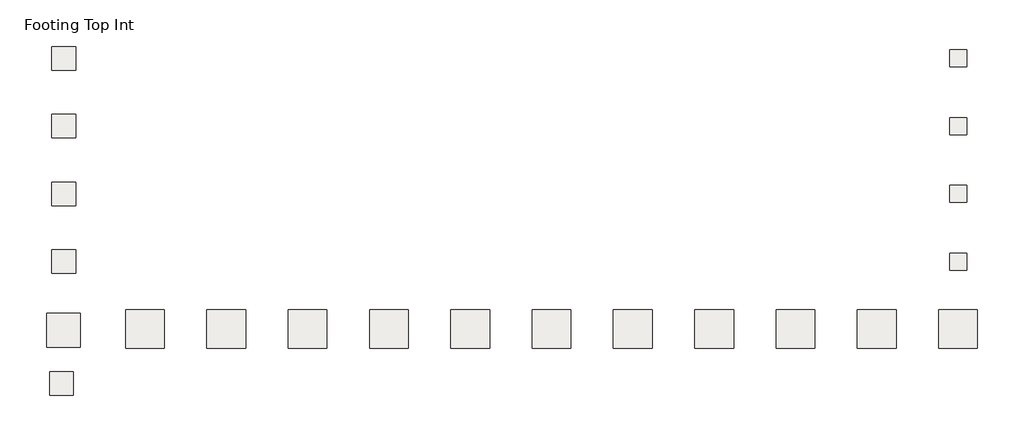
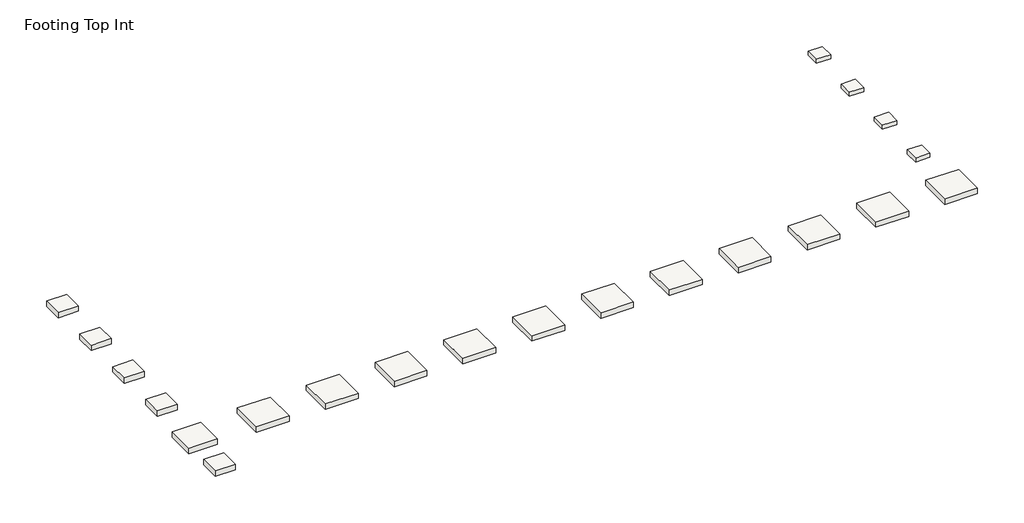
# One storey: 21 slabs.
"""IFC4 building model written with IfcOpenShell, lengths in millimetres."""

from ifc_helpers import new_model, si_unit, frame, origin, place, context, project, spatial, polyline, outline, extrude, element, save

model = new_model("IFC4")

# Units and contexts
model_context = context("Model", 3, world=origin())
ifc_project = project(units=[si_unit("LENGTHUNIT", "METRE", prefix="MILLI")], contexts=[model_context])

# Site, building, storey
site = spatial("IfcSite", under=ifc_project)
building = spatial("IfcBuilding", under=site)
storey = spatial("IfcBuildingStorey", under=building, Name="Footing Top Int", Elevation=-304.8)

# Slabs
placement = place(None, origin())
element("IfcSlab", 1, ObjectType="Footing-Rectangular : F10", at=placement, inside=storey, context=model_context, shape_type="SweptSolid", body=[
    extrude(outline(polyline([(321699.0398264, -566249.8913841), (324747.0398264, -566249.8913841), (324747.0398264, -569297.8913841), (321699.0398264, -569297.8913841), (321699.0398264, -566249.8913841)])), frame((0.0, 0.0, -914.4), z_axis=(0.0, 0.0, 1.0), x_axis=(1.0, 0.0, 0.0)), (0.0, 0.0, 1.0), 609.6),
])
element("IfcSlab", 2, ObjectType="Footing-Rectangular : F11", at=placement, inside=storey, context=model_context, shape_type="SweptSolid", body=[
    extrude(outline(polyline([(328849.1398264, -565913.3414082), (332354.3398264, -565913.3414082), (332354.3398264, -569418.5414082), (328849.1398264, -569418.5414082), (328849.1398264, -565913.3414082)])), frame((0.0, 0.0, -914.4), z_axis=(0.0, 0.0, 1.0), x_axis=(1.0, 0.0, 0.0)), (0.0, 0.0, 1.0), 609.6),
])
element("IfcSlab", 3, ObjectType="Footing-Rectangular : F11", at=placement, inside=storey, context=model_context, shape_type="SweptSolid", body=[
    extrude(outline(polyline([(336202.4398264, -565913.3414082), (339707.6398264, -565913.3414082), (339707.6398264, -569418.5414082), (336202.4398264, -569418.5414082), (336202.4398264, -565913.3414082)])), frame((0.0, 0.0, -914.4), z_axis=(0.0, 0.0, 1.0), x_axis=(1.0, 0.0, 0.0)), (0.0, 0.0, 1.0), 609.6),
])
element("IfcSlab", 4, ObjectType="Footing-Rectangular : F11", at=placement, inside=storey, context=model_context, shape_type="SweptSolid", body=[
    extrude(outline(polyline([(343555.7398264, -565913.3414082), (347060.9398264, -565913.3414082), (347060.9398264, -569418.5414082), (343555.7398264, -569418.5414082), (343555.7398264, -565913.3414082)])), frame((0.0, 0.0, -914.4), z_axis=(0.0, 0.0, 1.0), x_axis=(1.0, 0.0, 0.0)), (0.0, 0.0, 1.0), 609.6),
])
element("IfcSlab", 5, ObjectType="Footing-Rectangular : F11", at=placement, inside=storey, context=model_context, shape_type="SweptSolid", body=[
    extrude(outline(polyline([(350909.0398264, -565913.3414082), (354414.2398264, -565913.3414082), (354414.2398264, -569418.5414082), (350909.0398264, -569418.5414082), (350909.0398264, -565913.3414082)])), frame((0.0, 0.0, -914.4), z_axis=(0.0, 0.0, 1.0), x_axis=(1.0, 0.0, 0.0)), (0.0, 0.0, 1.0), 609.6),
])
element("IfcSlab", 6, ObjectType="Footing-Rectangular : F11", at=placement, inside=storey, context=model_context, shape_type="SweptSolid", body=[
    extrude(outline(polyline([(358262.3398264, -565913.3414082), (361767.5398264, -565913.3414082), (361767.5398264, -569418.5414082), (358262.3398264, -569418.5414082), (358262.3398264, -565913.3414082)])), frame((0.0, 0.0, -914.4), z_axis=(0.0, 0.0, 1.0), x_axis=(1.0, 0.0, 0.0)), (0.0, 0.0, 1.0), 609.6),
])
element("IfcSlab", 7, ObjectType="Footing-Rectangular : F11", at=placement, inside=storey, context=model_context, shape_type="SweptSolid", body=[
    extrude(outline(polyline([(365615.6398264, -565913.3414082), (369120.8398264, -565913.3414082), (369120.8398264, -569418.5414082), (365615.6398264, -569418.5414082), (365615.6398264, -565913.3414082)])), frame((0.0, 0.0, -914.4), z_axis=(0.0, 0.0, 1.0), x_axis=(1.0, 0.0, 0.0)), (0.0, 0.0, 1.0), 609.6),
])
element("IfcSlab", 8, ObjectType="Footing-Rectangular : F11", at=placement, inside=storey, context=model_context, shape_type="SweptSolid", body=[
    extrude(outline(polyline([(372968.9398264, -565913.3414082), (376474.1398264, -565913.3414082), (376474.1398264, -569418.5414082), (372968.9398264, -569418.5414082), (372968.9398264, -565913.3414082)])), frame((0.0, 0.0, -914.4), z_axis=(0.0, 0.0, 1.0), x_axis=(1.0, 0.0, 0.0)), (0.0, 0.0, 1.0), 609.6),
])
element("IfcSlab", 9, ObjectType="Footing-Rectangular : F11", at=placement, inside=storey, context=model_context, shape_type="SweptSolid", body=[
    extrude(outline(polyline([(380322.2398264, -565913.3414082), (383827.4398264, -565913.3414082), (383827.4398264, -569418.5414082), (380322.2398264, -569418.5414082), (380322.2398264, -565913.3414082)])), frame((0.0, 0.0, -914.4), z_axis=(0.0, 0.0, 1.0), x_axis=(1.0, 0.0, 0.0)), (0.0, 0.0, 1.0), 609.6),
])
element("IfcSlab", 10, ObjectType="Footing-Rectangular : F11", at=placement, inside=storey, context=model_context, shape_type="SweptSolid", body=[
    extrude(outline(polyline([(387675.5398264, -565913.3414082), (391180.7398264, -565913.3414082), (391180.7398264, -569418.5414082), (387675.5398264, -569418.5414082), (387675.5398264, -565913.3414082)])), frame((0.0, 0.0, -914.4), z_axis=(0.0, 0.0, 1.0), x_axis=(1.0, 0.0, 0.0)), (0.0, 0.0, 1.0), 609.6),
])
element("IfcSlab", 11, ObjectType="Footing-Rectangular : F11", at=placement, inside=storey, context=model_context, shape_type="SweptSolid", body=[
    extrude(outline(polyline([(395028.8398264, -565913.3414082), (398534.0398264, -565913.3414082), (398534.0398264, -569418.5414082), (395028.8398264, -569418.5414082), (395028.8398264, -565913.3414082)])), frame((0.0, 0.0, -914.4), z_axis=(0.0, 0.0, 1.0), x_axis=(1.0, 0.0, 0.0)), (0.0, 0.0, 1.0), 609.6),
])
element("IfcSlab", 12, ObjectType="Footing-Rectangular : F11", at=placement, inside=storey, context=model_context, shape_type="SweptSolid", body=[
    extrude(outline(polyline([(402382.1398264, -565913.3414082), (405887.3398264, -565913.3414082), (405887.3398264, -569418.5414082), (402382.1398264, -569418.5414082), (402382.1398264, -565913.3414082)])), frame((0.0, 0.0, -914.4), z_axis=(0.0, 0.0, 1.0), x_axis=(1.0, 0.0, 0.0)), (0.0, 0.0, 1.0), 609.6),
])
element("IfcSlab", 13, ObjectType="Footing-Rectangular : F5", at=placement, inside=storey, context=model_context, shape_type="SweptSolid", body=[
    extrude(outline(polyline([(404896.7398264, -542418.3413841), (404896.7398264, -543942.3413841), (403372.7398264, -543942.3413841), (403372.7398264, -542418.3413841), (404896.7398264, -542418.3413841)])), frame((0.0, 0.0, -762.0), z_axis=(0.0, 0.0, 1.0), x_axis=(1.0, 0.0, 0.0)), (0.0, 0.0, 1.0), 457.2),
])
element("IfcSlab", 14, ObjectType="Footing-Rectangular : F5", at=placement, inside=storey, context=model_context, shape_type="SweptSolid", body=[
    extrude(outline(polyline([(404896.7398264, -548546.0913841), (404896.7398264, -550070.0913841), (403372.7398264, -550070.0913841), (403372.7398264, -548546.0913841), (404896.7398264, -548546.0913841)])), frame((0.0, 0.0, -762.0), z_axis=(0.0, 0.0, 1.0), x_axis=(1.0, 0.0, 0.0)), (0.0, 0.0, 1.0), 457.2),
])
element("IfcSlab", 15, ObjectType="Footing-Rectangular : F5", at=placement, inside=storey, context=model_context, shape_type="SweptSolid", body=[
    extrude(outline(polyline([(404896.7398264, -554673.8413841), (404896.7398264, -556197.8413841), (403372.7398264, -556197.8413841), (403372.7398264, -554673.8413841), (404896.7398264, -554673.8413841)])), frame((0.0, 0.0, -762.0), z_axis=(0.0, 0.0, 1.0), x_axis=(1.0, 0.0, 0.0)), (0.0, 0.0, 1.0), 457.2),
])
element("IfcSlab", 16, ObjectType="Footing-Rectangular : F5", at=placement, inside=storey, context=model_context, shape_type="SweptSolid", body=[
    extrude(outline(polyline([(404896.7398264, -560801.5913841), (404896.7398264, -562325.5913841), (403372.7398264, -562325.5913841), (403372.7398264, -560801.5913841), (404896.7398264, -560801.5913841)])), frame((0.0, 0.0, -762.0), z_axis=(0.0, 0.0, 1.0), x_axis=(1.0, 0.0, 0.0)), (0.0, 0.0, 1.0), 457.2),
])
element("IfcSlab", 17, ObjectType="Footing-Rectangular : F7", at=placement, inside=storey, context=model_context, shape_type="SweptSolid", body=[
    extrude(outline(polyline([(324121.5648264, -571526.7413841), (324121.5648264, -573660.3413841), (321987.9648264, -573660.3413841), (321987.9648264, -571526.7413841), (324121.5648264, -571526.7413841)])), frame((0.0, 0.0, -914.4), z_axis=(0.0, 0.0, 1.0), x_axis=(1.0, 0.0, 0.0)), (0.0, 0.0, 1.0), 609.6),
])
element("IfcSlab", 18, ObjectType="Footing-Rectangular : F7", at=placement, inside=storey, context=model_context, shape_type="SweptSolid", body=[
    extrude(outline(polyline([(324324.7648264, -542113.5413841), (324324.7648264, -544247.1413841), (322191.1648264, -544247.1413841), (322191.1648264, -542113.5413841), (324324.7648264, -542113.5413841)])), frame((0.0, 0.0, -914.4), z_axis=(0.0, 0.0, 1.0), x_axis=(1.0, 0.0, 0.0)), (0.0, 0.0, 1.0), 609.6),
])
element("IfcSlab", 19, ObjectType="Footing-Rectangular : F7", at=placement, inside=storey, context=model_context, shape_type="SweptSolid", body=[
    extrude(outline(polyline([(324324.7648264, -548241.2913841), (324324.7648264, -550374.8913841), (322191.1648264, -550374.8913841), (322191.1648264, -548241.2913841), (324324.7648264, -548241.2913841)])), frame((0.0, 0.0, -914.4), z_axis=(0.0, 0.0, 1.0), x_axis=(1.0, 0.0, 0.0)), (0.0, 0.0, 1.0), 609.6),
])
element("IfcSlab", 20, ObjectType="Footing-Rectangular : F7", at=placement, inside=storey, context=model_context, shape_type="SweptSolid", body=[
    extrude(outline(polyline([(324324.7648264, -554369.0413841), (324324.7648264, -556502.6413841), (322191.1648264, -556502.6413841), (322191.1648264, -554369.0413841), (324324.7648264, -554369.0413841)])), frame((0.0, 0.0, -914.4), z_axis=(0.0, 0.0, 1.0), x_axis=(1.0, 0.0, 0.0)), (0.0, 0.0, 1.0), 609.6),
])
element("IfcSlab", 21, ObjectType="Footing-Rectangular : F7", at=placement, inside=storey, context=model_context, shape_type="SweptSolid", body=[
    extrude(outline(polyline([(324324.7648264, -560496.7913841), (324324.7648264, -562630.3913841), (322191.1648264, -562630.3913841), (322191.1648264, -560496.7913841), (324324.7648264, -560496.7913841)])), frame((0.0, 0.0, -914.4), z_axis=(0.0, 0.0, 1.0), x_axis=(1.0, 0.0, 0.0)), (0.0, 0.0, 1.0), 609.6),
])

save(model, "model.ifc")

# Revit data of these elements
# Type "Footing-Rectangular : F10"
#   Assembly Code = "A1010100"
#   Width = 10' - 0"
#   Length = 10' - 0"
#   Thickness = 2' - 0"
#   Structural Material [instance default] = CONCRETE FOOTING - SEE STRUCT DWGS.
# Type "Footing-Rectangular : F11"
#   Assembly Code = "A1010100"
#   Width = 11' - 6"
#   Length = 11' - 6"
#   Thickness = 2' - 0"
#   Structural Material [instance default] = CONCRETE FOOTING - SEE STRUCT DWGS.
# Type "Footing-Rectangular : F5"
#   Assembly Code = "A1010100"
#   Width = 5' - 0"
#   Length = 5' - 0"
#   Thickness = 1' - 6"
#   Structural Material [instance default] = CONCRETE FOOTING - SEE STRUCT DWGS.
# Type "Footing-Rectangular : F7"
#   Assembly Code = "A1010100"
#   Width = 7' - 0"
#   Length = 7' - 0"
#   Thickness = 2' - 0"
#   Structural Material [instance default] = CONCRETE FOOTING - SEE STRUCT DWGS.
# Element 1 (IfcSlab, "Footing-Rectangular : F10")
#   Comments = ""
#   Structural Material = CONCRETE FOOTING - SEE STRUCT DWGS.
#   Phase Created = Existing
#   Materials on its faces: "CONCRETE FOOTING - SEE STRUCT DWGS."
# Elements 2, 3, 4, 5, 6, 7, 8, 9, 10, 11, 12 (IfcSlab, "Footing-Rectangular : F11")
#   Comments = ""
#   Structural Material = CONCRETE FOOTING - SEE STRUCT DWGS.
#   Phase Created = Existing
#   Materials on its faces: "CONCRETE FOOTING - SEE STRUCT DWGS."
# Elements 13, 14, 15, 16 (IfcSlab, "Footing-Rectangular : F5")
#   Comments = ""
#   Structural Material = CONCRETE FOOTING - SEE STRUCT DWGS.
#   Phase Created = Existing
#   Materials on its faces: "CONCRETE FOOTING - SEE STRUCT DWGS."
# Elements 17, 18, 19, 20, 21 (IfcSlab, "Footing-Rectangular : F7")
#   Comments = ""
#   Structural Material = CONCRETE FOOTING - SEE STRUCT DWGS.
#   Phase Created = Existing
#   Materials on its faces: "CONCRETE FOOTING - SEE STRUCT DWGS."
# Materials
#   "CONCRETE FOOTING - SEE STRUCT DWGS.": class "Concrete", colour RGB 192 192 192, transparency 0, Description = "Cast-in-place concrete", Cost = 0
